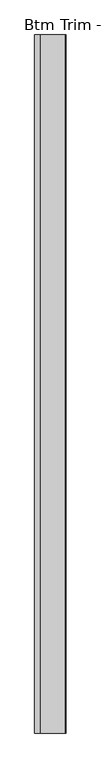
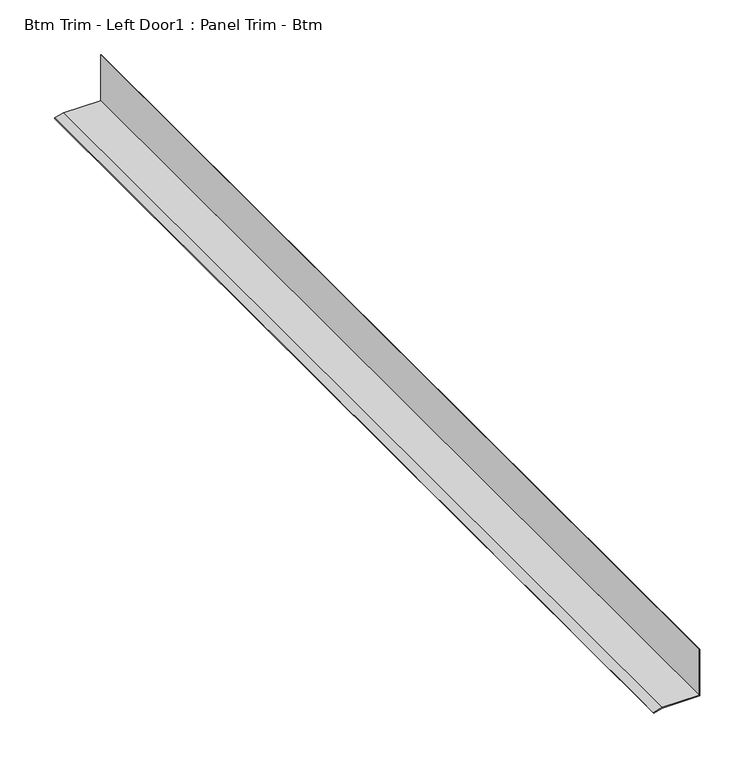
"""IFC4 building model written with IfcOpenShell, lengths in millimetres: proxy geometry, Btm Trim - Left Door1 : Panel Trim - Btm."""

from ifc_helpers import new_model, si_unit, frame, origin, place, context, project, spatial, polyline, outline, extrude, source, transform, mapped, element, save


def btm_trim_left_door1_panel_trim_btm_e3873032(model_context):
    return source(origin(), model_context, "Body", "SweptSolid", [
        extrude(outline(polyline([(50.8, 587326.1141748), (48.3077022, 587316.8127928), (47.5409986, 587317.0182304), (50.00625, 587326.2186739), (50.00625, 587365.8934739), (101.6, 587365.8934739), (101.6, 587365.1060739), (50.8, 587365.1060739), (50.8, 587326.1141748)])), frame((0.0, -535202.3537841, 0.0), z_axis=(0.0, 1.0, 0.0), x_axis=(0.0, 0.0, 1.0)), (0.0, 0.0, 1.0), 1093.7880247),
    ])


if __name__ == "__main__":
    model = new_model("IFC4")
    model_context = context("Model", 3, world=origin())
    ifc_project = project(units=[si_unit("LENGTHUNIT", "METRE", prefix="MILLI")], contexts=[model_context])
    site = spatial("IfcSite", under=ifc_project)
    building = spatial("IfcBuilding", under=site)
    placement = place(None, origin())
    btm_trim_left_door1_panel_trim_btm_shape = btm_trim_left_door1_panel_trim_btm_e3873032(model_context)
    element("IfcBuildingElementProxy", 1, Name="Btm Trim - Left Door1 : Panel Trim - Btm", ObjectType="Btm Trim - Left Door1 : Panel Trim - Btm", at=placement, inside=building, context=model_context, shape_type="MappedRepresentation", body=[
        mapped(btm_trim_left_door1_panel_trim_btm_shape, transform((0.0, 0.0, 0.0), x_axis=(1.0, 0.0, 0.0), y_axis=(0.0, 1.0, 0.0), z_axis=(0.0, 0.0, 1.0))),
    ])
    save(model, "model.ifc")

# Revit data of these elements
# Element 1 (IfcBuildingElementProxy, "Btm Trim - Left Door1 : Panel Trim - Btm")
#   Materials on its faces: "BASE TRIM BY MTL PANEL MFR."
# Materials
#   "BASE TRIM BY MTL PANEL MFR.": class "Generic", colour RGB 239 242 240, transparency 0, Cost = 0
